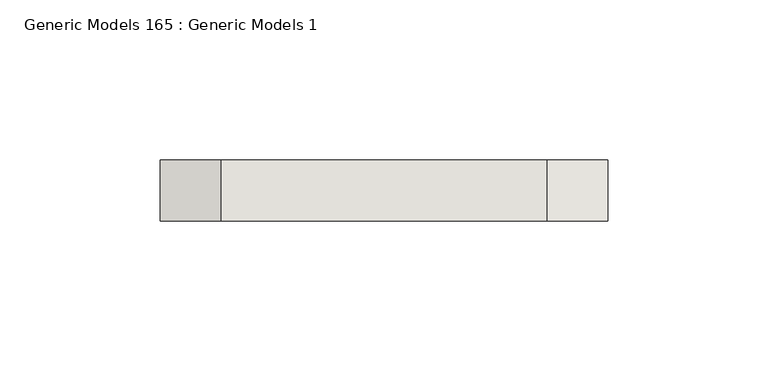
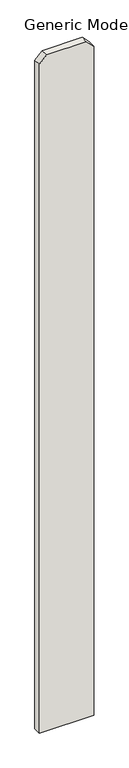
"""IFC4 building model written with IfcOpenShell, lengths in millimetres: wall geometry, Generic Models 165 : Generic Models 1."""

import ifcopenshell
import ifcopenshell.guid

model = None  # the IFC model being written
_history = None  # IfcOwnerHistory: only IFC2X3 demands one
_inside = {}  # id of a spatial element -> (the spatial element, [elements in it])
_under = {}  # id of a project, library or spatial element -> (it, [spatial elements below it])
_declared = {}  # id of a project -> (the project, [libraries it declares])
_typed = {}  # id of a type object -> (the type object, [elements of that type])
_made_of = {}  # id of a material, layer set ... -> (it, [elements and type objects made of it])


def new_model(schema):
    """Start an empty IFC model of exactly this schema.

    Asked for "IFC4X3", IfcOpenShell would pick the latest addendum, in which some entities
    have other attributes; the version numbers below select the first issue.
    IFC2X3 requires an IfcOwnerHistory on every rooted entity: one is made here for all.
    """
    global model, _history
    if schema == "IFC4X3":
        model = ifcopenshell.file(schema_version=(4, 3, 0, 0))
    else:
        model = ifcopenshell.file(schema=schema)
    _inside.clear()
    _under.clear()
    _declared.clear()
    _typed.clear()
    _made_of.clear()
    _history = None
    if model.schema == "IFC2X3":
        org = make("IfcOrganization", Name="unknown")
        user = make(
            "IfcPersonAndOrganization",
            ThePerson=make("IfcPerson", FamilyName="unknown"),
            TheOrganization=org,
        )
        app = make(
            "IfcApplication",
            ApplicationDeveloper=org,
            Version="unknown",
            ApplicationFullName="unknown",
            ApplicationIdentifier="unknown",
        )
        _history = make(
            "IfcOwnerHistory",
            OwningUser=user,
            OwningApplication=app,
            ChangeAction="ADDED",
            CreationDate=0,
        )
    return model


def make(cls, **values):
    """One entity of the class cls with the attributes given. An attribute that is None is left unset."""
    return model.create_entity(
        cls, **{name: value for name, value in values.items() if value is not None}
    )


def rooted(cls, **values):
    """An entity with a GlobalId (a new one), such as an element, a storey or a relation."""
    return make(cls, GlobalId=ifcopenshell.guid.new(), OwnerHistory=_history, **values)


def si_unit(unit_type, name, prefix=None):
    """IfcSIUnit, for example si_unit("LENGTHUNIT", "METRE", prefix="MILLI")."""
    return make("IfcSIUnit", UnitType=unit_type, Prefix=prefix, Name=name)


def assignment(units):
    """IfcUnitAssignment: the units of a project."""
    return None if units is None else make("IfcUnitAssignment", Units=units)


def point(xyz):
    """IfcCartesianPoint."""
    return None if xyz is None else make("IfcCartesianPoint", Coordinates=xyz)


def direction(xyz):
    """IfcDirection."""
    return None if xyz is None else make("IfcDirection", DirectionRatios=xyz)


def frame(location, z_axis=None, x_axis=None):
    """IfcAxis2Placement3D, a coordinate frame: its origin and axes. An axis left out is left unset."""
    return make(
        "IfcAxis2Placement3D",
        Location=point(location),
        Axis=direction(z_axis),
        RefDirection=direction(x_axis),
    )


def origin():
    """The frame at (0, 0, 0) with its axes left unset."""
    return frame((0.0, 0.0, 0.0))


def place(relative_to, where):
    """IfcLocalPlacement: puts the frame where relative to a parent placement (None: the world)."""
    return make(
        "IfcLocalPlacement", PlacementRelTo=relative_to, RelativePlacement=where
    )


def context(
    kind, dimensions, precision=None, world=None, true_north=None, identifier=None
):
    """IfcGeometricRepresentationContext, for example the 3D "Model" context."""
    return make(
        "IfcGeometricRepresentationContext",
        ContextIdentifier=identifier,
        ContextType=kind,
        CoordinateSpaceDimension=dimensions,
        Precision=precision,
        WorldCoordinateSystem=world,
        TrueNorth=true_north,
    )


def project(units=None, contexts=None):
    """IfcProject with its units and contexts."""
    return rooted(
        "IfcProject",
        Name="project",
        RepresentationContexts=contexts,
        UnitsInContext=assignment(units),
    )


def spatial(cls, under=None, at=None, **own):
    """A site, building, storey or space (cls), placed at a placement, below another one or the project."""
    s = rooted(cls, ObjectPlacement=at, **own)
    if under is not None:
        _under.setdefault(under.id(), (under, []))[1].append(s)
    return s


def polyline(points):
    """IfcPolyline through the points."""
    return make("IfcPolyline", Points=[point(p) for p in points])


def outline(outer, holes=None, kind="AREA"):
    """IfcArbitraryClosedProfileDef: a profile drawn as a closed curve; with holes, ...WithVoids."""
    if holes is None:
        return make("IfcArbitraryClosedProfileDef", ProfileType=kind, OuterCurve=outer)
    return make(
        "IfcArbitraryProfileDefWithVoids",
        ProfileType=kind,
        OuterCurve=outer,
        InnerCurves=holes,
    )


def extrude(swept, where, along, depth):
    """IfcExtrudedAreaSolid: the profile swept, set in the frame where, extruded along a direction by depth."""
    return make(
        "IfcExtrudedAreaSolid",
        SweptArea=swept,
        Position=where,
        ExtrudedDirection=direction(along),
        Depth=depth,
    )


def shape(context_of_items, identifier, shape_type, items):
    """IfcShapeRepresentation: the items that make up one representation, for example the "Body"."""
    return make(
        "IfcShapeRepresentation",
        ContextOfItems=context_of_items,
        RepresentationIdentifier=identifier,
        RepresentationType=shape_type,
        Items=items,
    )


def source(mapping_origin, context_of_items, identifier, shape_type, items):
    """IfcRepresentationMap: a shape defined once, which mapped items show again and again."""
    return make(
        "IfcRepresentationMap",
        MappingOrigin=mapping_origin,
        MappedRepresentation=shape(context_of_items, identifier, shape_type, items),
    )


def transform(
    local_origin,
    x_axis=None,
    y_axis=None,
    z_axis=None,
    scale=None,
    scale2=None,
    scale3=None,
    uniform=True,
):
    """IfcCartesianTransformationOperator3D, or its non-uniform kind. x_axis, y_axis, z_axis: its Axis1, 2, 3."""
    if uniform:
        return make(
            "IfcCartesianTransformationOperator3D",
            Axis1=direction(x_axis),
            Axis2=direction(y_axis),
            LocalOrigin=point(local_origin),
            Scale=scale,
            Axis3=direction(z_axis),
        )
    return make(
        "IfcCartesianTransformationOperator3DnonUniform",
        Axis1=direction(x_axis),
        Axis2=direction(y_axis),
        LocalOrigin=point(local_origin),
        Scale=scale,
        Axis3=direction(z_axis),
        Scale2=scale2,
        Scale3=scale3,
    )


def mapped(mapping_source, mapping_target):
    """IfcMappedItem: shows the shape of a source again, moved by a transform."""
    return make(
        "IfcMappedItem", MappingSource=mapping_source, MappingTarget=mapping_target
    )


def made_of(thing, what):
    """Note that an element or type object is made of a material, layer set ...; save() writes the relation."""
    if what is not None:
        _made_of.setdefault(what.id(), (what, []))[1].append(thing)
    return thing


def element(
    cls,
    number,
    at=None,
    inside=None,
    cuts=None,
    type_object=None,
    material=None,
    context=None,
    identifier="Body",
    shape_type=None,
    held_by="IfcProductDefinitionShape",
    body=None,
    shapes=None,
    **own,
):
    """One element of the class cls, such as IfcWall. Its Tag is "e" and its number.

    at: its placement. inside: the storey or other place that contains it. cuts: it is an
    opening in that element (IfcRelVoidsElement). A single representation is given by context,
    identifier, shape_type and body (its items); several are given by shapes. held_by: the class
    of the entity that holds the representations. save() writes the other relations.
    """
    e = rooted(cls, Tag="e%d" % number, ObjectPlacement=at, **own)
    if body is not None:
        shapes = [shape(context, identifier, shape_type, body)]
    if shapes is not None:
        e.Representation = make(held_by, Representations=shapes)
    if inside is not None:
        _inside.setdefault(inside.id(), (inside, []))[1].append(e)
    if cuts is not None:
        rooted(
            "IfcRelVoidsElement", RelatingBuildingElement=cuts, RelatedOpeningElement=e
        )
    if type_object is not None:
        _typed.setdefault(type_object.id(), (type_object, []))[1].append(e)
    return made_of(e, material)


def aggregate(whole, parts):
    """IfcRelAggregates: a whole, such as a stair, and the parts it consists of."""
    return rooted("IfcRelAggregates", RelatingObject=whole, RelatedObjects=parts)


def save(model, path):
    """Write the relations noted so far, then the file.

    IfcRelAggregates (storeys below a building ...), IfcRelContainedInSpatialStructure (elements
    in a storey), IfcRelDefinesByType, IfcRelAssociatesMaterial and IfcRelDeclares: one each for
    every whole, place, type object, material and project.
    """
    for whole, parts in _under.values():
        aggregate(whole, parts)
    for where, things in _inside.values():
        rooted(
            "IfcRelContainedInSpatialStructure",
            RelatedElements=things,
            RelatingStructure=where,
        )
    for kind, things in _typed.values():
        rooted("IfcRelDefinesByType", RelatedObjects=things, RelatingType=kind)
    for what, things in _made_of.values():
        rooted("IfcRelAssociatesMaterial", RelatedObjects=things, RelatingMaterial=what)
    for by, libraries in _declared.values():
        rooted("IfcRelDeclares", RelatingContext=by, RelatedDefinitions=libraries)
    model.write(path)


def generic_models_165_generic_models_1_e4cc997e(model_context):
    return source(origin(), model_context, "Body", "SweptSolid", [
        extrude(outline(polyline([(76.2, 324127.8125), (1885.95, 324127.8125), (1905.0, 324108.7625), (1905.0, 324007.1625), (1885.95, 323988.1125), (76.2, 323988.1125), (76.2, 324127.8125)])), frame((0.0, 547.6875, 0.0), z_axis=(0.0, 1.0, 0.0), x_axis=(0.0, 0.0, 1.0)), (0.0, 0.0, 1.0), 19.05),
    ])


if __name__ == "__main__":
    model = new_model("IFC4")
    model_context = context("Model", 3, world=origin())
    ifc_project = project(units=[si_unit("LENGTHUNIT", "METRE", prefix="MILLI")], contexts=[model_context])
    site = spatial("IfcSite", under=ifc_project)
    building = spatial("IfcBuilding", under=site)
    placement = place(None, origin())
    generic_models_165_generic_models_1_shape = generic_models_165_generic_models_1_e4cc997e(model_context)
    element("IfcWall", 1, ObjectType="Generic Models 165 : Generic Models 1", at=placement, inside=building, context=model_context, shape_type="MappedRepresentation", body=[
        mapped(generic_models_165_generic_models_1_shape, transform((0.0, 0.0, 0.0), x_axis=(1.0, 0.0, 0.0), y_axis=(0.0, 1.0, 0.0), z_axis=(0.0, 0.0, 1.0))),
    ])
    save(model, "model.ifc")

# Revit data of these elements
# Element 1 (IfcWall, "Generic Models 165 : Generic Models 1")
#   Materials on its faces: "VERTICAL 1X6 CEDAR PLANKS W/ CLEAR WOOD SEALER"
# Materials
#   "VERTICAL 1X6 CEDAR PLANKS W/ CLEAR WOOD SEALER": class "Wood", colour RGB 234 198 147, transparency 0, Description = "Pinus Echinata", Cost = 0
